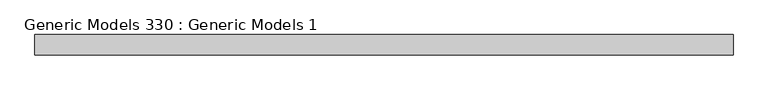
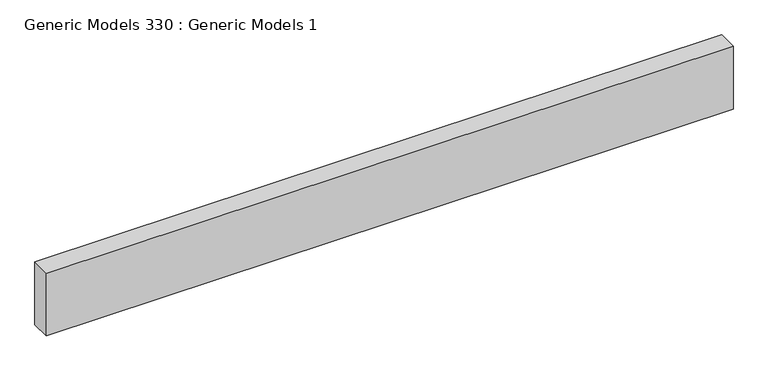
"""IFC4 building model written with IfcOpenShell, lengths in millimetres: proxy geometry, Generic Models 330 : Generic Models 1."""

from ifc_helpers import new_model, si_unit, frame, origin, place, context, project, spatial, polyline, outline, extrude, source, transform, mapped, element, save


def generic_models_330_generic_models_1_196bba55(model_context):
    return source(origin(), model_context, "Body", "SweptSolid", [
        extrude(outline(polyline([(-9254.0286296, -4113.4499282), (-9254.0286296, -4037.2499282), (-6623.9669063, -4037.2499282), (-6623.9669063, -4113.4499282), (-9254.0286296, -4113.4499282)])), frame((0.0, 0.0, 126415.546), z_axis=(0.0, 0.0, 1.0), x_axis=(1.0, 0.0, 0.0)), (0.0, 0.0, 1.0), 254.0),
    ])


if __name__ == "__main__":
    model = new_model("IFC4")
    model_context = context("Model", 3, world=origin())
    ifc_project = project(units=[si_unit("LENGTHUNIT", "METRE", prefix="MILLI")], contexts=[model_context])
    site = spatial("IfcSite", under=ifc_project)
    building = spatial("IfcBuilding", under=site)
    placement = place(None, origin())
    generic_models_330_generic_models_1_shape = generic_models_330_generic_models_1_196bba55(model_context)
    element("IfcBuildingElementProxy", 1, Name="Generic Models 330 : Generic Models 1", ObjectType="Generic Models 330 : Generic Models 1", at=placement, inside=building, context=model_context, shape_type="MappedRepresentation", body=[
        mapped(generic_models_330_generic_models_1_shape, transform((0.0, 0.0, 0.0), x_axis=(1.0, 0.0, 0.0), y_axis=(0.0, 1.0, 0.0), z_axis=(0.0, 0.0, 1.0))),
    ])
    save(model, "model.ifc")

# Revit data of these elements
# Element 1 (IfcBuildingElementProxy, "Generic Models 330 : Generic Models 1")
#   Materials on its faces: "_STRUCTURAL MEMBER (SEE STRUCT. DWGS)"
# Materials
#   "_STRUCTURAL MEMBER (SEE STRUCT. DWGS)": class "Generic", colour RGB 209 182 141, transparency 0, Cost = 0
